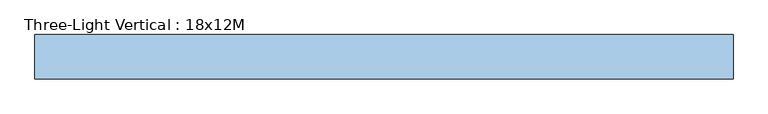
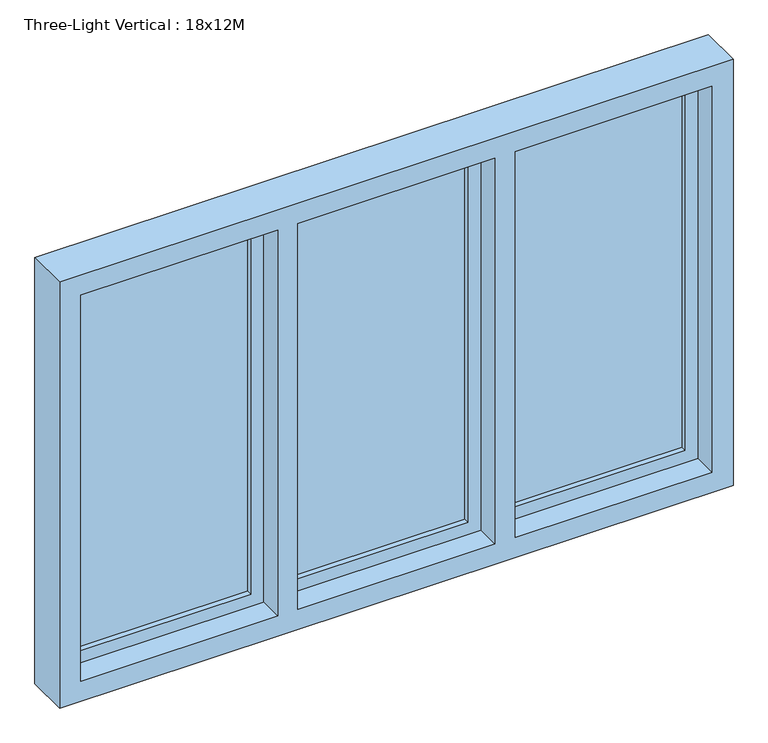
"""IFC4 building model written with IfcOpenShell, lengths in millimetres: window geometry, Three-Light Vertical : 18x12M."""

import ifcopenshell
import ifcopenshell.guid

model = None  # the IFC model being written
_history = None  # IfcOwnerHistory: only IFC2X3 demands one
_inside = {}  # id of a spatial element -> (the spatial element, [elements in it])
_under = {}  # id of a project, library or spatial element -> (it, [spatial elements below it])
_declared = {}  # id of a project -> (the project, [libraries it declares])
_typed = {}  # id of a type object -> (the type object, [elements of that type])
_made_of = {}  # id of a material, layer set ... -> (it, [elements and type objects made of it])


def new_model(schema):
    """Start an empty IFC model of exactly this schema.

    Asked for "IFC4X3", IfcOpenShell would pick the latest addendum, in which some entities
    have other attributes; the version numbers below select the first issue.
    IFC2X3 requires an IfcOwnerHistory on every rooted entity: one is made here for all.
    """
    global model, _history
    if schema == "IFC4X3":
        model = ifcopenshell.file(schema_version=(4, 3, 0, 0))
    else:
        model = ifcopenshell.file(schema=schema)
    _inside.clear()
    _under.clear()
    _declared.clear()
    _typed.clear()
    _made_of.clear()
    _history = None
    if model.schema == "IFC2X3":
        org = make("IfcOrganization", Name="unknown")
        user = make(
            "IfcPersonAndOrganization",
            ThePerson=make("IfcPerson", FamilyName="unknown"),
            TheOrganization=org,
        )
        app = make(
            "IfcApplication",
            ApplicationDeveloper=org,
            Version="unknown",
            ApplicationFullName="unknown",
            ApplicationIdentifier="unknown",
        )
        _history = make(
            "IfcOwnerHistory",
            OwningUser=user,
            OwningApplication=app,
            ChangeAction="ADDED",
            CreationDate=0,
        )
    return model


def make(cls, **values):
    """One entity of the class cls with the attributes given. An attribute that is None is left unset."""
    return model.create_entity(
        cls, **{name: value for name, value in values.items() if value is not None}
    )


def rooted(cls, **values):
    """An entity with a GlobalId (a new one), such as an element, a storey or a relation."""
    return make(cls, GlobalId=ifcopenshell.guid.new(), OwnerHistory=_history, **values)


def si_unit(unit_type, name, prefix=None):
    """IfcSIUnit, for example si_unit("LENGTHUNIT", "METRE", prefix="MILLI")."""
    return make("IfcSIUnit", UnitType=unit_type, Prefix=prefix, Name=name)


def assignment(units):
    """IfcUnitAssignment: the units of a project."""
    return None if units is None else make("IfcUnitAssignment", Units=units)


def point(xyz):
    """IfcCartesianPoint."""
    return None if xyz is None else make("IfcCartesianPoint", Coordinates=xyz)


def direction(xyz):
    """IfcDirection."""
    return None if xyz is None else make("IfcDirection", DirectionRatios=xyz)


def frame(location, z_axis=None, x_axis=None):
    """IfcAxis2Placement3D, a coordinate frame: its origin and axes. An axis left out is left unset."""
    return make(
        "IfcAxis2Placement3D",
        Location=point(location),
        Axis=direction(z_axis),
        RefDirection=direction(x_axis),
    )


def origin():
    """The frame at (0, 0, 0) with its axes left unset."""
    return frame((0.0, 0.0, 0.0))


def place(relative_to, where):
    """IfcLocalPlacement: puts the frame where relative to a parent placement (None: the world)."""
    return make(
        "IfcLocalPlacement", PlacementRelTo=relative_to, RelativePlacement=where
    )


def context(
    kind, dimensions, precision=None, world=None, true_north=None, identifier=None
):
    """IfcGeometricRepresentationContext, for example the 3D "Model" context."""
    return make(
        "IfcGeometricRepresentationContext",
        ContextIdentifier=identifier,
        ContextType=kind,
        CoordinateSpaceDimension=dimensions,
        Precision=precision,
        WorldCoordinateSystem=world,
        TrueNorth=true_north,
    )


def project(units=None, contexts=None):
    """IfcProject with its units and contexts."""
    return rooted(
        "IfcProject",
        Name="project",
        RepresentationContexts=contexts,
        UnitsInContext=assignment(units),
    )


def spatial(cls, under=None, at=None, **own):
    """A site, building, storey or space (cls), placed at a placement, below another one or the project."""
    s = rooted(cls, ObjectPlacement=at, **own)
    if under is not None:
        _under.setdefault(under.id(), (under, []))[1].append(s)
    return s


def polyline(points):
    """IfcPolyline through the points."""
    return make("IfcPolyline", Points=[point(p) for p in points])


def outline(outer, holes=None, kind="AREA"):
    """IfcArbitraryClosedProfileDef: a profile drawn as a closed curve; with holes, ...WithVoids."""
    if holes is None:
        return make("IfcArbitraryClosedProfileDef", ProfileType=kind, OuterCurve=outer)
    return make(
        "IfcArbitraryProfileDefWithVoids",
        ProfileType=kind,
        OuterCurve=outer,
        InnerCurves=holes,
    )


def extrude(swept, where, along, depth):
    """IfcExtrudedAreaSolid: the profile swept, set in the frame where, extruded along a direction by depth."""
    return make(
        "IfcExtrudedAreaSolid",
        SweptArea=swept,
        Position=where,
        ExtrudedDirection=direction(along),
        Depth=depth,
    )


def faces_of(points, faces, orient=None, outer=None):
    """IfcFace entities. A face is a list of loops; a loop is a list of indices into points, from 0.

    orient and outer hold one flag for each loop. By default every Orientation is true, the
    first loop of a face is its IfcFaceOuterBound and the others are IfcFaceBound.
    """
    made = []
    for i, loops in enumerate(faces):
        bounds = []
        for j, loop in enumerate(loops):
            is_outer = j == 0 if outer is None else outer[i][j]
            bounds.append(
                make(
                    "IfcFaceOuterBound" if is_outer else "IfcFaceBound",
                    Bound=make("IfcPolyLoop", Polygon=[points[k] for k in loop]),
                    Orientation=True if orient is None else orient[i][j],
                )
            )
        made.append(make("IfcFace", Bounds=bounds))
    return made


def faceted_brep(points, faces, orient=None, outer=None, voids=None):
    """IfcFacetedBrep: a solid bounded by flat faces; with voids (closed shells), ...WithVoids."""
    shared = [point(p) for p in points]
    hull = make("IfcClosedShell", CfsFaces=faces_of(shared, faces, orient, outer))
    if voids is None:
        return make("IfcFacetedBrep", Outer=hull)
    return make(
        "IfcFacetedBrepWithVoids",
        Outer=hull,
        Voids=[
            make(cls, CfsFaces=faces_of(shared, fs, o, b)) for cls, fs, o, b in voids
        ],
    )


def shape(context_of_items, identifier, shape_type, items):
    """IfcShapeRepresentation: the items that make up one representation, for example the "Body"."""
    return make(
        "IfcShapeRepresentation",
        ContextOfItems=context_of_items,
        RepresentationIdentifier=identifier,
        RepresentationType=shape_type,
        Items=items,
    )


def source(mapping_origin, context_of_items, identifier, shape_type, items):
    """IfcRepresentationMap: a shape defined once, which mapped items show again and again."""
    return make(
        "IfcRepresentationMap",
        MappingOrigin=mapping_origin,
        MappedRepresentation=shape(context_of_items, identifier, shape_type, items),
    )


def transform(
    local_origin,
    x_axis=None,
    y_axis=None,
    z_axis=None,
    scale=None,
    scale2=None,
    scale3=None,
    uniform=True,
):
    """IfcCartesianTransformationOperator3D, or its non-uniform kind. x_axis, y_axis, z_axis: its Axis1, 2, 3."""
    if uniform:
        return make(
            "IfcCartesianTransformationOperator3D",
            Axis1=direction(x_axis),
            Axis2=direction(y_axis),
            LocalOrigin=point(local_origin),
            Scale=scale,
            Axis3=direction(z_axis),
        )
    return make(
        "IfcCartesianTransformationOperator3DnonUniform",
        Axis1=direction(x_axis),
        Axis2=direction(y_axis),
        LocalOrigin=point(local_origin),
        Scale=scale,
        Axis3=direction(z_axis),
        Scale2=scale2,
        Scale3=scale3,
    )


def mapped(mapping_source, mapping_target):
    """IfcMappedItem: shows the shape of a source again, moved by a transform."""
    return make(
        "IfcMappedItem", MappingSource=mapping_source, MappingTarget=mapping_target
    )


def made_of(thing, what):
    """Note that an element or type object is made of a material, layer set ...; save() writes the relation."""
    if what is not None:
        _made_of.setdefault(what.id(), (what, []))[1].append(thing)
    return thing


def element(
    cls,
    number,
    at=None,
    inside=None,
    cuts=None,
    type_object=None,
    material=None,
    context=None,
    identifier="Body",
    shape_type=None,
    held_by="IfcProductDefinitionShape",
    body=None,
    shapes=None,
    **own,
):
    """One element of the class cls, such as IfcWall. Its Tag is "e" and its number.

    at: its placement. inside: the storey or other place that contains it. cuts: it is an
    opening in that element (IfcRelVoidsElement). A single representation is given by context,
    identifier, shape_type and body (its items); several are given by shapes. held_by: the class
    of the entity that holds the representations. save() writes the other relations.
    """
    e = rooted(cls, Tag="e%d" % number, ObjectPlacement=at, **own)
    if body is not None:
        shapes = [shape(context, identifier, shape_type, body)]
    if shapes is not None:
        e.Representation = make(held_by, Representations=shapes)
    if inside is not None:
        _inside.setdefault(inside.id(), (inside, []))[1].append(e)
    if cuts is not None:
        rooted(
            "IfcRelVoidsElement", RelatingBuildingElement=cuts, RelatedOpeningElement=e
        )
    if type_object is not None:
        _typed.setdefault(type_object.id(), (type_object, []))[1].append(e)
    return made_of(e, material)


def aggregate(whole, parts):
    """IfcRelAggregates: a whole, such as a stair, and the parts it consists of."""
    return rooted("IfcRelAggregates", RelatingObject=whole, RelatedObjects=parts)


def save(model, path):
    """Write the relations noted so far, then the file.

    IfcRelAggregates (storeys below a building ...), IfcRelContainedInSpatialStructure (elements
    in a storey), IfcRelDefinesByType, IfcRelAssociatesMaterial and IfcRelDeclares: one each for
    every whole, place, type object, material and project.
    """
    for whole, parts in _under.values():
        aggregate(whole, parts)
    for where, things in _inside.values():
        rooted(
            "IfcRelContainedInSpatialStructure",
            RelatedElements=things,
            RelatingStructure=where,
        )
    for kind, things in _typed.values():
        rooted("IfcRelDefinesByType", RelatedObjects=things, RelatingType=kind)
    for what, things in _made_of.values():
        rooted("IfcRelAssociatesMaterial", RelatedObjects=things, RelatingMaterial=what)
    for by, libraries in _declared.values():
        rooted("IfcRelDeclares", RelatingContext=by, RelatedDefinitions=libraries)
    model.write(path)


def three_light_vertical_18x12m_b3fc569e(model_context):
    return source(origin(), model_context, "Body", "SolidModel", [
        extrude(outline(polyline([(1970.0, -924.0), (842.0, -924.0), (842.0, -364.6666667), (1970.0, -364.6666667), (1970.0, -924.0)]), holes=[polyline([(1920.0, -414.6666667), (892.0, -414.6666667), (892.0, -874.0), (1920.0, -874.0), (1920.0, -414.6666667)])]), frame((0.0, 134.0, 0.0), z_axis=(0.0, 1.0, 0.0), x_axis=(0.0, 0.0, 1.0)), (0.0, 0.0, 1.0), 50.0),
        extrude(outline(polyline([(1970.0, -339.6666667), (842.0, -339.6666667), (842.0, 219.6666667), (1970.0, 219.6666667), (1970.0, -339.6666667)]), holes=[polyline([(1920.0, 169.6666667), (892.0, 169.6666667), (892.0, -289.6666667), (1920.0, -289.6666667), (1920.0, 169.6666667)])]), frame((0.0, 134.0, 0.0), z_axis=(0.0, 1.0, 0.0), x_axis=(0.0, 0.0, 1.0)), (0.0, 0.0, 1.0), 50.0),
        extrude(outline(polyline([(1970.0, 244.6666667), (842.0, 244.6666667), (842.0, 804.0), (1970.0, 804.0), (1970.0, 244.6666667)]), holes=[polyline([(1920.0, 754.0), (892.0, 754.0), (892.0, 294.6666667), (1920.0, 294.6666667), (1920.0, 754.0)])]), frame((0.0, 134.0, 0.0), z_axis=(0.0, 1.0, 0.0), x_axis=(0.0, 0.0, 1.0)), (0.0, 0.0, 1.0), 50.0),
        faceted_brep([(-966.0, 184.0, 800.0), (846.0, 184.0, 800.0), (846.0, 69.0, 800.0), (-966.0, 69.0, 800.0), (846.0, 184.0, 2012.0), (846.0, 69.0, 2012.0), (-966.0, 184.0, 2012.0), (804.0, 184.0, 842.0), (804.0, 184.0, 1970.0), (244.6666667, 184.0, 1970.0), (244.6666667, 184.0, 842.0), (-924.0, 184.0, 1970.0), (-924.0, 184.0, 842.0), (-364.6666667, 184.0, 842.0), (-364.6666667, 184.0, 1970.0), (219.6666667, 184.0, 1970.0), (-339.6666667, 184.0, 1970.0), (-339.6666667, 184.0, 842.0), (219.6666667, 184.0, 842.0), (-966.0, 69.0, 2012.0), (789.0, 69.0, 1955.0), (789.0, 69.0, 857.0), (259.6666667, 69.0, 857.0), (259.6666667, 69.0, 1955.0), (204.6666667, 69.0, 857.0), (-324.6666667, 69.0, 857.0), (-324.6666667, 69.0, 1955.0), (204.6666667, 69.0, 1955.0), (-909.0, 69.0, 857.0), (-909.0, 69.0, 1955.0), (-379.6666667, 69.0, 1955.0), (-379.6666667, 69.0, 857.0), (789.0, 134.0, 857.0), (259.6666667, 134.0, 857.0), (-909.0, 134.0, 857.0), (-379.6666667, 134.0, 857.0), (204.6666667, 134.0, 857.0), (-324.6666667, 134.0, 857.0), (789.0, 134.0, 1955.0), (804.0, 134.0, 1970.0), (804.0, 134.0, 842.0), (244.6666667, 134.0, 842.0), (244.6666667, 134.0, 1970.0), (259.6666667, 134.0, 1955.0), (-924.0, 134.0, 842.0), (-924.0, 134.0, 1970.0), (-364.6666667, 134.0, 1970.0), (-364.6666667, 134.0, 842.0), (-909.0, 134.0, 1955.0), (-379.6666667, 134.0, 1955.0), (219.6666667, 134.0, 1970.0), (219.6666667, 134.0, 842.0), (-339.6666667, 134.0, 842.0), (-339.6666667, 134.0, 1970.0), (204.6666667, 134.0, 1955.0), (-324.6666667, 134.0, 1955.0)], [[[0, 1, 2, 3]], [[2, 1, 4, 5]], [[4, 1, 0, 6], [7, 8, 9, 10], [11, 12, 13, 14], [15, 16, 17, 18]], [[2, 5, 19, 3], [20, 21, 22, 23], [24, 25, 26, 27], [28, 29, 30, 31]], [[21, 32, 33, 22]], [[34, 28, 31, 35]], [[24, 36, 37, 25]], [[32, 21, 20, 38]], [[39, 40, 41, 42], [32, 38, 43, 33]], [[44, 45, 46, 47], [48, 34, 35, 49]], [[50, 51, 52, 53], [36, 54, 55, 37]], [[52, 51, 18, 17]], [[40, 7, 10, 41]], [[12, 44, 47, 13]], [[7, 40, 39, 8]], [[19, 6, 0, 3]], [[48, 29, 28, 34]], [[11, 45, 44, 12]], [[10, 9, 42, 41]], [[23, 22, 33, 43]], [[24, 27, 54, 36]], [[15, 18, 51, 50]], [[17, 16, 53, 52]], [[26, 25, 37, 55]], [[31, 30, 49, 35]], [[14, 13, 47, 46]], [[19, 5, 4, 6]], [[38, 20, 23, 43]], [[29, 48, 49, 30]], [[54, 27, 26, 55]], [[8, 39, 42, 9]], [[15, 50, 53, 16]], [[46, 45, 11, 14]]]),
        extrude(outline(polyline([(-289.6666667, 170.0), (169.6666667, 170.0), (169.6666667, 148.0), (-289.6666667, 148.0), (-289.6666667, 170.0)])), frame((0.0, 0.0, 892.0), z_axis=(0.0, 0.0, 1.0), x_axis=(1.0, 0.0, 0.0)), (0.0, 0.0, 1.0), 1028.0),
        extrude(outline(polyline([(-874.0, 170.0), (-414.6666667, 170.0), (-414.6666667, 148.0), (-874.0, 148.0), (-874.0, 170.0)])), frame((0.0, 0.0, 892.0), z_axis=(0.0, 0.0, 1.0), x_axis=(1.0, 0.0, 0.0)), (0.0, 0.0, 1.0), 1028.0),
        extrude(outline(polyline([(294.6666667, 170.0), (754.0, 170.0), (754.0, 148.0), (294.6666667, 148.0), (294.6666667, 170.0)])), frame((0.0, 0.0, 892.0), z_axis=(0.0, 0.0, 1.0), x_axis=(1.0, 0.0, 0.0)), (0.0, 0.0, 1.0), 1028.0),
    ])


if __name__ == "__main__":
    model = new_model("IFC4")
    model_context = context("Model", 3, world=origin())
    ifc_project = project(units=[si_unit("LENGTHUNIT", "METRE", prefix="MILLI")], contexts=[model_context])
    site = spatial("IfcSite", under=ifc_project)
    building = spatial("IfcBuilding", under=site)
    placement = place(None, origin())
    three_light_vertical_18x12m_shape = three_light_vertical_18x12m_b3fc569e(model_context)
    element("IfcWindow", 1, ObjectType="Three-Light Vertical : 18x12M", at=placement, inside=building, context=model_context, shape_type="MappedRepresentation", body=[
        mapped(three_light_vertical_18x12m_shape, transform((0.0, 0.0, 0.0), x_axis=(1.0, 0.0, 0.0), y_axis=(0.0, 1.0, 0.0), z_axis=(0.0, 0.0, 1.0))),
    ])
    save(model, "model.ifc")

# Revit data of these elements
# Type "Three-Light Vertical : 18x12M"
#   Type Mark = "50"
#   Creator Organization [instance default] = "© Danish Educational Content"
#   Creator Name [instance default] = "© Erik Falck Jørgensen"
#   Creator Build [instance default] = "2017.0801.0"
#   Analytic Construction = "<None>"
#   length#6 = -36 mm
#   length#5 = -14 mm
#   length#4 = 120 mm
#   length#3 = 29.5 mm
#   length#2 = 57 mm
#   length#1 = 0 mm
#   Seal Width = 12 mm
#   Rough Width = 1812 mm
#   Rough Height = 1212 mm
#   Rebate Depth = 50 mm
#   Transom Width = 55 mm
#   Rabbet Width = 15 mm
#   Rabbet Depth = 50 mm
#   Height = 1188 mm
#   Glass Thickness = 22 mm
#   Frame Width = 50 mm
#   Frame Depth = 50 mm
#   Exterior Direction [instance default] = 0.00°
#   Case Depth = 115 mm
#   Case Width = 45 mm
#   Default Sill Height = 800 mm
#   Width = 1788 mm
#   Sealing = no
#   Hinging = yes
#   Wall Closure = 1
#   Above Cutplane [instance default] = no
#   Glass = none
#   Case/Transom = none
#   Frame/Mullion = none
#   Assembly Code = ""
# Element 1 (IfcWindow, "Three-Light Vertical : 18x12M")
#   Materials on its faces: "Default Frame/Mullion (Interior/Exterior)", "Glass"
# Materials
#   "Default Frame/Mullion (Interior/Exterior)": class "Generic", colour RGB 205 205 205, transparency 0, Description = "Udefineret karm/ramme materiale", Cost = 0
#   "Glass": class "Glass", colour RGB 180 200 255, transparency 0.75, Description = "Generisk glas", Cost = 0
